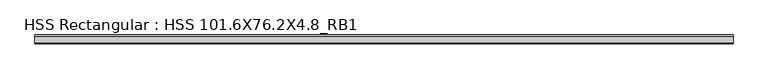
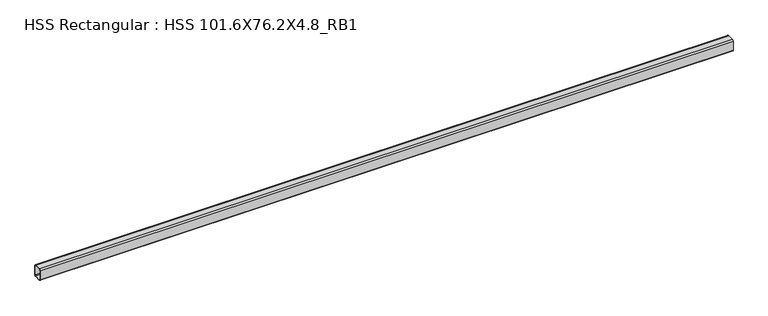
"""IFC4 building model written with IfcOpenShell, lengths in millimetres: beam geometry, HSS Rectangular : HSS 101.6X76.2X4.8_RB1."""

from ifc_helpers import new_model, si_unit, point, frame, frame_2d, origin, place, context, project, spatial, polyline, circle_curve, trimmed, segment, composite_curve, outline, extrude, source, transform, mapped, element, save


def hss_rectangular_hss_101_6x76_2x4_8_rb1_e6dae79d(model_context):
    return source(origin(), model_context, "Body", "SweptSolid", [
        extrude(outline(composite_curve([segment(polyline([(38.1, 41.275), (38.1, -41.275)]), True, "CONTINUOUS"), segment(trimmed(circle_curve(frame_2d((28.575, -41.275)), 9.525), [point((38.1, -41.275))], [point((28.575, -50.8))], False, "CARTESIAN"), True, "CONTINUOUS"), segment(polyline([(28.575, -50.8), (-28.575, -50.8)]), True, "CONTINUOUS"), segment(trimmed(circle_curve(frame_2d((-28.575, -41.275)), 9.525), [point((-28.575, -50.8))], [point((-38.1, -41.275))], False, "CARTESIAN"), True, "CONTINUOUS"), segment(polyline([(-38.1, -41.275), (-38.1, 41.275)]), True, "CONTINUOUS"), segment(trimmed(circle_curve(frame_2d((-28.575, 41.275)), 9.525), [point((-38.1, 41.275))], [point((-28.575, 50.8))], False, "CARTESIAN"), True, "CONTINUOUS"), segment(polyline([(-28.575, 50.8), (28.575, 50.8)]), True, "CONTINUOUS"), segment(trimmed(circle_curve(frame_2d((28.575, 41.275)), 9.525), [point((28.575, 50.8))], [point((38.1, 41.275))], False, "CARTESIAN"), True, "CONTINUOUS")], self_intersect=False), holes=[composite_curve([segment(trimmed(circle_curve(frame_2d((-28.575, 41.275)), 4.7625), [point((-28.575, 46.0375))], [point((-33.3375, 41.275))], True, "CARTESIAN"), True, "CONTINUOUS"), segment(polyline([(-33.3375, 41.275), (-33.3375, -41.275)]), True, "CONTINUOUS"), segment(trimmed(circle_curve(frame_2d((-28.575, -41.275)), 4.7625), [point((-33.3375, -41.275))], [point((-28.575, -46.0375))], True, "CARTESIAN"), True, "CONTINUOUS"), segment(polyline([(-28.575, -46.0375), (28.575, -46.0375)]), True, "CONTINUOUS"), segment(trimmed(circle_curve(frame_2d((28.575, -41.275)), 4.7625), [point((28.575, -46.0375))], [point((33.3375, -41.275))], True, "CARTESIAN"), True, "CONTINUOUS"), segment(polyline([(33.3375, -41.275), (33.3375, 41.275)]), True, "CONTINUOUS"), segment(trimmed(circle_curve(frame_2d((28.575, 41.275)), 4.7625), [point((33.3375, 41.275))], [point((28.575, 46.0375))], True, "CARTESIAN"), True, "CONTINUOUS"), segment(polyline([(28.575, 46.0375), (-28.575, 46.0375)]), True, "CONTINUOUS")], self_intersect=False)]), frame((-7500.0, 0.0, 0.0), z_axis=(1.0, 0.0, 0.0), x_axis=(0.0, 1.0, 0.0)), (0.0, 0.0, 1.0), 5946.0149745),
    ])


if __name__ == "__main__":
    model = new_model("IFC4")
    model_context = context("Model", 3, world=origin())
    ifc_project = project(units=[si_unit("LENGTHUNIT", "METRE", prefix="MILLI")], contexts=[model_context])
    site = spatial("IfcSite", under=ifc_project)
    building = spatial("IfcBuilding", under=site)
    placement = place(None, origin())
    hss_rectangular_hss_101_6x76_2x4_8_rb1_shape = hss_rectangular_hss_101_6x76_2x4_8_rb1_e6dae79d(model_context)
    element("IfcBeam", 1, ObjectType="HSS Rectangular : HSS 101.6X76.2X4.8_RB1", at=placement, inside=building, context=model_context, shape_type="MappedRepresentation", body=[
        mapped(hss_rectangular_hss_101_6x76_2x4_8_rb1_shape, transform((0.0, 0.0, 0.0), x_axis=(1.0, 0.0, 0.0), y_axis=(0.0, 1.0, 0.0), z_axis=(0.0, 0.0, 1.0))),
    ])
    save(model, "model.ifc")

# Revit data of these elements
# Type "HSS Rectangular : HSS 101.6X76.2X4.8_RB1"
#   Section Name Key = "HSS 4X3X3/16"
#   Assembly Code = "B10"
#   Width = 7.62 cm
#   Wall Nominal Thickness = 0.4763 cm
#   Wall Design Thickness = 0.442 cm
#   Torsional Moment of Inertia = 260.561 cm⁴
#   Torsional Modulus = 61.2876 cm³
#   Section Area = 14.4516 cm²
#   Plastic Modulus weak axis = 40.3122 cm³
#   Plastic Modulus strong axis = 49.1612 cm³
#   Perimeter = 0.881482 m²/m
#   Outer Fillet = 0.9525 cm
#   Nominal Weight = 12.1285 kgf/m
#   Moment of Inertia weak axis = 131.529 cm⁴
#   Moment of Inertia strong axis = 205.202 cm⁴
#   Inner Fillet = 0.4763 cm
#   Height = 10.16 cm
#   Elastic Modulus weak axis = 34.4128 cm³
#   Elastic Modulus strong axis = 40.476 cm³
#   Centroid Vertical = 5.08 cm
#   Centroid Horizontal = 3.81 cm
#   Length [instance default] = 1524 mm
#   Structural Material [instance default] = Steel ASTM A500, Grade B, Rectangular and Square
#   Principal Axes Angle = 0
# Element 1 (IfcBeam, "HSS Rectangular : HSS 101.6X76.2X4.8_RB1")
#   Structural Material = Steel ASTM A992
#   Materials on its faces: "Steel ASTM A992"
# Materials
#   "Steel ASTM A500, Grade B, Rectangular and Square": class "Metal", colour RGB 199 199 199, transparency 0, Description = "Carbon steel", Cost = 0
#   "Steel ASTM A992": class "Metal", colour RGB 199 199 199, transparency 0, Description = "Structural steel 50ksi", Cost = 0
